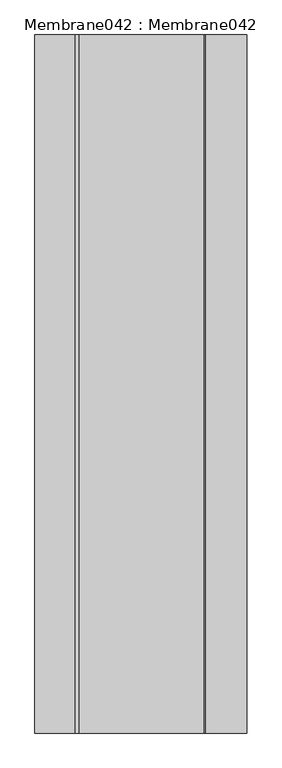
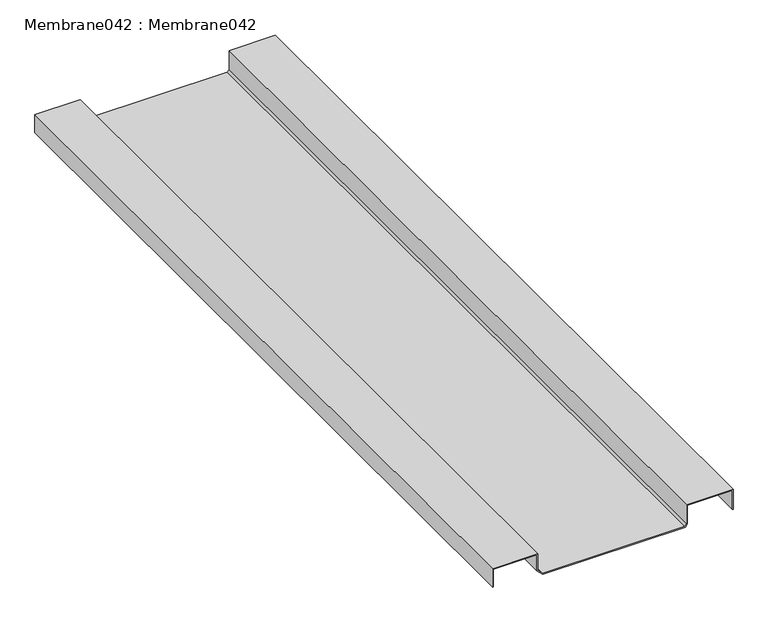
"""IFC4 building model written with IfcOpenShell, lengths in millimetres: proxy geometry, Membrane042 : Membrane042."""

from ifc_helpers import new_model, si_unit, frame, origin, place, context, project, spatial, polyline, outline, extrude, source, transform, mapped, element, save


def membrane042_membrane042_a91ebf19(model_context):
    return source(origin(), model_context, "Body", "SweptSolid", [
        extrude(outline(polyline([(40111.328125, -9288.9824219), (40163.8320313, -9288.9824219), (40163.8320313, -9406.2119141), (40112.7345471, -9406.2119141), (40107.5625, -9410.821371), (40107.5625, -9768.9815951), (40120.3582916, -9782.1787109), (40164.75, -9782.1787109), (40164.75, -9896.0849609), (40115.640625, -9896.0849609), (40115.640625, -9894.0849609), (40162.75, -9894.0849609), (40162.75, -9784.1787109), (40119.5117187, -9784.1787109), (40105.5625, -9769.7919922), (40105.5625, -9409.9248047), (40111.9726562, -9404.2119141), (40161.8320312, -9404.2119141), (40161.8320312, -9290.9824219), (40111.328125, -9290.9824219), (40111.328125, -9288.9824219)])), frame((0.0, 7982.1531721, 0.0), z_axis=(0.0, 1.0, 0.0), x_axis=(0.0, 0.0, 1.0)), (0.0, 0.0, 1.0), 2000.0),
    ])


if __name__ == "__main__":
    model = new_model("IFC4")
    model_context = context("Model", 3, world=origin())
    ifc_project = project(units=[si_unit("LENGTHUNIT", "METRE", prefix="MILLI")], contexts=[model_context])
    site = spatial("IfcSite", under=ifc_project)
    building = spatial("IfcBuilding", under=site)
    placement = place(None, origin())
    membrane042_membrane042_shape = membrane042_membrane042_a91ebf19(model_context)
    element("IfcBuildingElementProxy", 1, Name="Membrane042 : Membrane042", ObjectType="Membrane042 : Membrane042", at=placement, inside=building, context=model_context, shape_type="MappedRepresentation", body=[
        mapped(membrane042_membrane042_shape, transform((0.0, 0.0, 0.0), x_axis=(1.0, 0.0, 0.0), y_axis=(0.0, 1.0, 0.0), z_axis=(0.0, 0.0, 1.0))),
    ])
    save(model, "model.ifc")

# Revit data of these elements
# Type "Membrane042 : Membrane042"
#   NameOverride = "Membrane042"
# Element 1 (IfcBuildingElementProxy, "Membrane042 : Membrane042")
#   Materials on its faces: "WESTCOAT ALX UNDER TILE WATERPROOFING SYSTEM (FOLLOW MANUFACTURER'S INSTALLATION REQUIREMENTS)"
# Materials
#   "WESTCOAT ALX UNDER TILE WATERPROOFING SYSTEM (FOLLOW MANUFACTURER'S INSTALLATION REQUIREMENTS)": class "Unassigned", colour RGB 27 232 0, transparency 0
